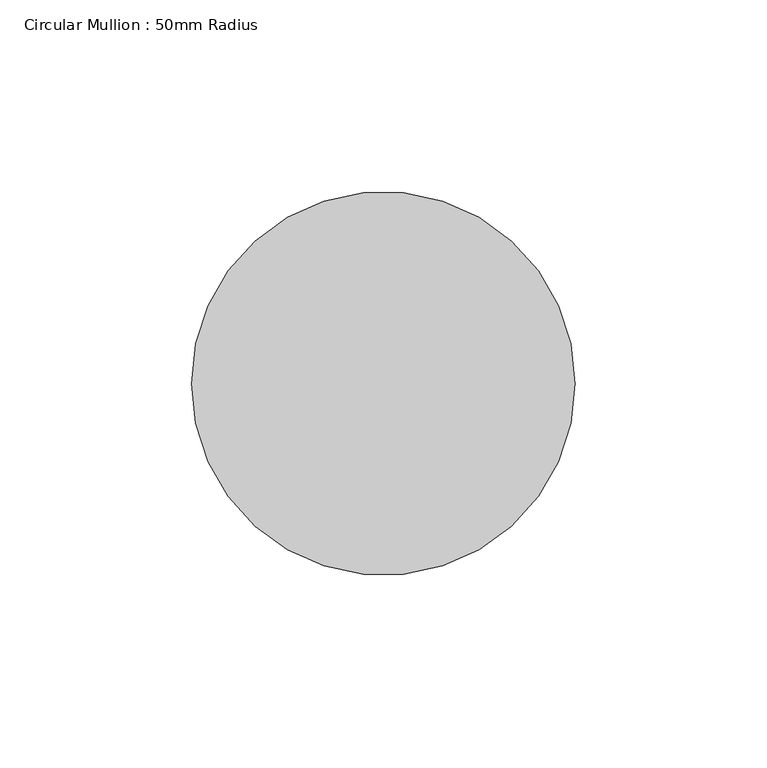
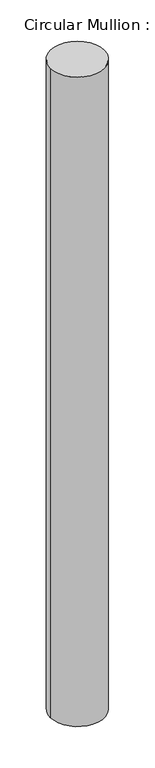
"""IFC4 building model written with IfcOpenShell, lengths in millimetres: member geometry, Circular Mullion : 50mm Radius."""

from ifc_helpers import new_model, si_unit, point, frame, origin, origin_2d, place, context, project, spatial, circle_curve, trimmed, segment, composite_curve, outline, extrude, source, transform, mapped, element, save


def circular_mullion_50mm_radius_dc219947(model_context):
    return source(origin(), model_context, "Body", "SweptSolid", [
        extrude(outline(composite_curve([segment(trimmed(circle_curve(origin_2d(), 50.0), [point((50.0, 0.0))], [point((-50.0, 0.0))], False, "CARTESIAN"), True, "CONTINUOUS"), segment(trimmed(circle_curve(origin_2d(), 50.0), [point((-50.0, 0.0))], [point((50.0, 0.0))], False, "CARTESIAN"), True, "CONTINUOUS")], self_intersect=False)), frame((0.0, 0.0, -1273.7209105), z_axis=(0.0, 0.0, 1.0), x_axis=(1.0, 0.0, 0.0)), (0.0, 0.0, 1.0), 1273.7209105),
    ])


if __name__ == "__main__":
    model = new_model("IFC4")
    model_context = context("Model", 3, world=origin())
    ifc_project = project(units=[si_unit("LENGTHUNIT", "METRE", prefix="MILLI")], contexts=[model_context])
    site = spatial("IfcSite", under=ifc_project)
    building = spatial("IfcBuilding", under=site)
    placement = place(None, origin())
    circular_mullion_50mm_radius_shape = circular_mullion_50mm_radius_dc219947(model_context)
    element("IfcMember", 1, ObjectType="Circular Mullion : 50mm Radius", at=placement, inside=building, context=model_context, shape_type="MappedRepresentation", body=[
        mapped(circular_mullion_50mm_radius_shape, transform((0.0, 0.0, 0.0), x_axis=(1.0, 0.0, 0.0), y_axis=(0.0, 1.0, 0.0), z_axis=(0.0, 0.0, 1.0))),
    ])
    save(model, "model.ifc")

# Revit data of these elements
# Type "Circular Mullion : 50mm Radius"
#   built-in parameter 1007350 = 0.164042 (stored number, unit not read)
# Element 1 (IfcMember, "Circular Mullion : 50mm Radius")
#   Materials on its faces: "Aluminium"
# Materials
#   "Aluminium": class "Metal", colour RGB 247 247 247, transparency 0, Description = "Aluminium 6061", Cost = 0
